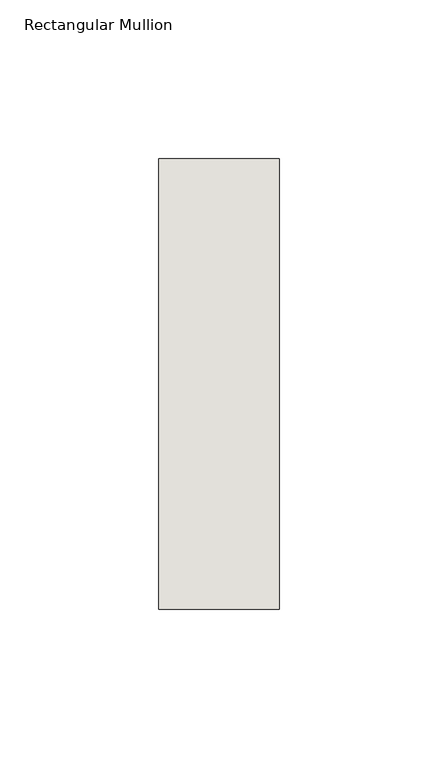
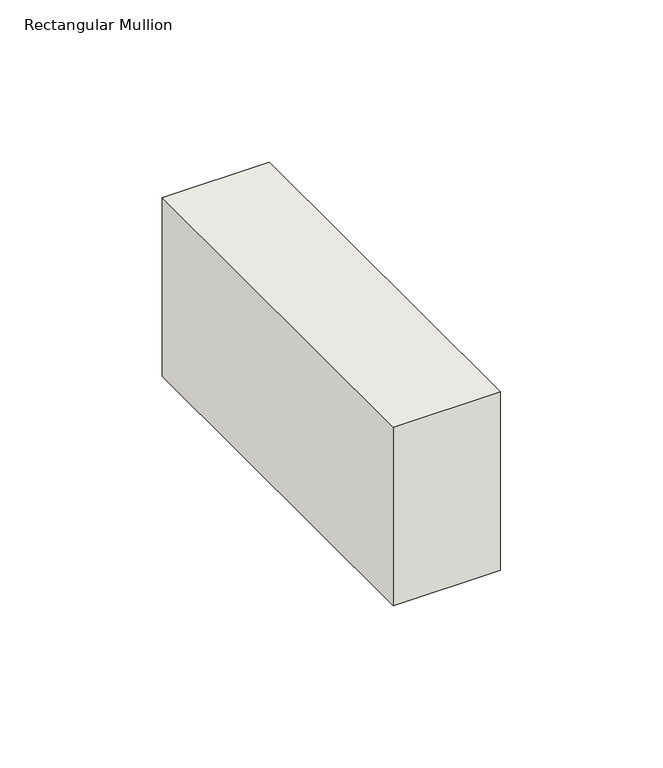
"""IFC4 building model written with IfcOpenShell, lengths in millimetres: wall geometry, Rectangular Mullion : NLRS_21_CWM_hsb-regel 38x142_gen_rsf."""

from ifc_helpers import new_model, si_unit, frame, origin, place, context, project, spatial, polyline, outline, extrude, source, transform, mapped, element, save


def rectangular_mullion_f185e772(model_context):
    return source(origin(), model_context, "Body", "SweptSolid", [
        extrude(outline(polyline([(0.0, -71.0), (-38.0, -71.0), (-38.0, 71.0), (0.0, 71.0), (0.0, -71.0)])), frame((0.0, 0.0, -66.9999997), z_axis=(0.0, 0.0, 1.0), x_axis=(1.0, 0.0, 0.0)), (0.0, 0.0, 1.0), 66.9999997),
    ])


if __name__ == "__main__":
    model = new_model("IFC4")
    model_context = context("Model", 3, world=origin())
    ifc_project = project(units=[si_unit("LENGTHUNIT", "METRE", prefix="MILLI")], contexts=[model_context])
    site = spatial("IfcSite", under=ifc_project)
    building = spatial("IfcBuilding", under=site)
    placement = place(None, origin())
    rectangular_mullion_shape = rectangular_mullion_f185e772(model_context)
    element("IfcWall", 1, ObjectType="Rectangular Mullion : NLRS_21_CWM_hsb-regel 38x142_gen_rsf", at=placement, inside=building, context=model_context, shape_type="MappedRepresentation", body=[
        mapped(rectangular_mullion_shape, transform((0.0, 0.0, 0.0), x_axis=(1.0, 0.0, 0.0), y_axis=(0.0, 1.0, 0.0), z_axis=(0.0, 0.0, 1.0))),
    ])
    save(model, "model.ifc")

# Revit data of these elements
# Type "Rectangular Mullion : NLRS_21_CWM_hsb-regel 38x142_gen_rsf"
#   Type IfcGUID = "07M7mRoiH1CR8m_RSKIwpF"
#   Assembly Code = "21.10"
#   IfcExportAs = "IfcWall"
#   built-in parameter 1007322 = 0.465879 (stored number, unit not read)
#   built-in parameter 1007321 = 0.062336 (stored number, unit not read)
#   built-in parameter 1007320 = 0.062336 (stored number, unit not read)
# Element 1 (IfcWall, "Rectangular Mullion : NLRS_21_CWM_hsb-regel 38x142_gen_rsf")
#   Materials on its faces: "NLRS_i2_hout naaldhout vuren_gen_rsf"
# Materials
#   "NLRS_i2_hout naaldhout vuren_gen_rsf": class "I - Hout", colour RGB 234 199 147, transparency 0, Keynote = "i2", Manufacturer = "Revit Standards Foundation", URL = "www.revitstandards.org", Description = "hout vuren", Cost = 0
